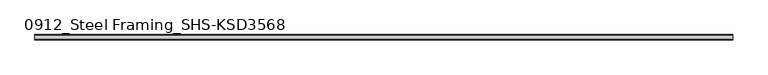
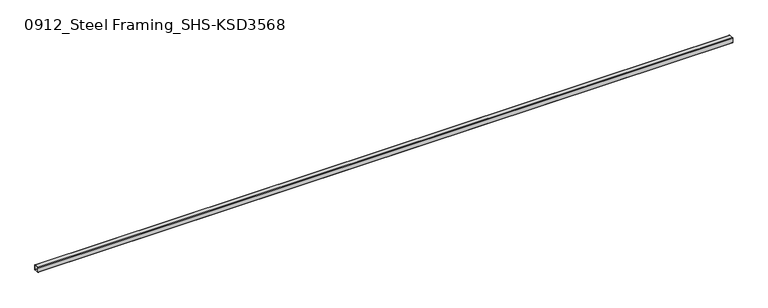
"""IFC4 building model written with IfcOpenShell, lengths in millimetres: beam geometry, 0912_Steel Framing_SHS-KSD3568 : H_SB_ASB_SHS-150x150x6."""

from ifc_helpers import new_model, si_unit, point, frame, frame_2d, origin, place, context, project, spatial, polyline, circle_curve, trimmed, segment, composite_curve, outline, extrude, source, transform, mapped, element, save


def beam_0912_steel_framing_shs_ksd3568_e683b74f(model_context):
    return source(origin(), model_context, "Body", "SweptSolid", [
        extrude(outline(composite_curve([segment(polyline([(75.0, 63.0), (75.0, -63.0)]), True, "CONTINUOUS"), segment(trimmed(circle_curve(frame_2d((63.0, -63.0)), 12.0), [point((75.0, -63.0))], [point((63.0, -75.0))], False, "CARTESIAN"), True, "CONTINUOUS"), segment(polyline([(63.0, -75.0), (-63.0, -75.0)]), True, "CONTINUOUS"), segment(trimmed(circle_curve(frame_2d((-63.0, -63.0)), 12.0), [point((-63.0, -75.0))], [point((-75.0, -63.0))], False, "CARTESIAN"), True, "CONTINUOUS"), segment(polyline([(-75.0, -63.0), (-75.0, 63.0)]), True, "CONTINUOUS"), segment(trimmed(circle_curve(frame_2d((-63.0, 63.0)), 12.0), [point((-75.0, 63.0))], [point((-63.0, 75.0))], False, "CARTESIAN"), True, "CONTINUOUS"), segment(polyline([(-63.0, 75.0), (63.0, 75.0)]), True, "CONTINUOUS"), segment(trimmed(circle_curve(frame_2d((63.0, 63.0)), 12.0), [point((63.0, 75.0))], [point((75.0, 63.0))], False, "CARTESIAN"), True, "CONTINUOUS")], self_intersect=False), holes=[composite_curve([segment(trimmed(circle_curve(frame_2d((-63.0, 63.0)), 6.0), [point((-63.0, 69.0))], [point((-69.0, 63.0))], True, "CARTESIAN"), True, "CONTINUOUS"), segment(polyline([(-69.0, 63.0), (-69.0, -63.0)]), True, "CONTINUOUS"), segment(trimmed(circle_curve(frame_2d((-63.0, -63.0)), 6.0), [point((-69.0, -63.0))], [point((-63.0, -69.0))], True, "CARTESIAN"), True, "CONTINUOUS"), segment(polyline([(-63.0, -69.0), (63.0, -69.0)]), True, "CONTINUOUS"), segment(trimmed(circle_curve(frame_2d((63.0, -63.0)), 6.0), [point((63.0, -69.0))], [point((69.0, -63.0))], True, "CARTESIAN"), True, "CONTINUOUS"), segment(polyline([(69.0, -63.0), (69.0, 63.0)]), True, "CONTINUOUS"), segment(trimmed(circle_curve(frame_2d((63.0, 63.0)), 6.0), [point((69.0, 63.0))], [point((63.0, 69.0))], True, "CARTESIAN"), True, "CONTINUOUS"), segment(polyline([(63.0, 69.0), (-63.0, 69.0)]), True, "CONTINUOUS")], self_intersect=False)]), frame((-9880.0, 0.0, 0.0), z_axis=(1.0, 0.0, 0.0), x_axis=(0.0, 1.0, 0.0)), (0.0, 0.0, 1.0), 19760.0),
    ])


if __name__ == "__main__":
    model = new_model("IFC4")
    model_context = context("Model", 3, world=origin())
    ifc_project = project(units=[si_unit("LENGTHUNIT", "METRE", prefix="MILLI")], contexts=[model_context])
    site = spatial("IfcSite", under=ifc_project)
    building = spatial("IfcBuilding", under=site)
    placement = place(None, origin())
    beam_0912_steel_framing_shs_ksd3568_shape = beam_0912_steel_framing_shs_ksd3568_e683b74f(model_context)
    element("IfcBeam", 1, ObjectType="0912_Steel Framing_SHS-KSD3568 : H_SB_ASB_SHS-150x150x6", at=placement, inside=building, context=model_context, shape_type="MappedRepresentation", body=[
        mapped(beam_0912_steel_framing_shs_ksd3568_shape, transform((0.0, 0.0, 0.0), x_axis=(1.0, 0.0, 0.0), y_axis=(0.0, 1.0, 0.0), z_axis=(0.0, 0.0, 1.0))),
    ])
    save(model, "model.ifc")

# Revit data of these elements
# Type "0912_Steel Framing_SHS-KSD3568 : H_SB_ASB_SHS-150x150x6"
#   H_WM Code_1 = "S01AA002-00001 | Main Steel Structure Fabrication Work | Shelter/Building | Medium Steel - Standard (90KG/M>Weight≥30KG/M) | Material: (   )"
#   H_WM Code_2 = "S03AA028-00001 | Main Steel Structure Erection Work | Shelter/Building | Medium Steel (90KG/M>Weight≥30KG/M) | Material: (   )"
#   H_WM Code_3 = "S01AA010-00001 | Main Steel Structure Fabrication Work | Shelter/Building | Steel Painting/Coating | for Non-Fireproofed Steel Surface, Surface Preparation, Primer, Second & Final Coat | Material: (   )"
#   H_Q'ty Cal Type Tag = "SB-Q2"
#   Perimeter = 0.60 m²/m
#   Nominal Weight = 26.40 kgf/m
#   Length [instance default] = 1.0000 m
#   b = 0.1500 m
#   h = 0.1500 m
#   tr = 0.0120 m
#   t = 0.0060 m
#   A = 28.36 m²
#   Structural Material [instance default] = Steel, 45-345
# Element 1 (IfcBeam, "0912_Steel Framing_SHS-KSD3568 : H_SB_ASB_SHS-150x150x6")
#   Structural Material = none
# Materials
#   "Steel, 45-345": class "Metal", colour RGB 189 187 185, transparency 0, Description = "Steel 345 MPa", Cost = 0
